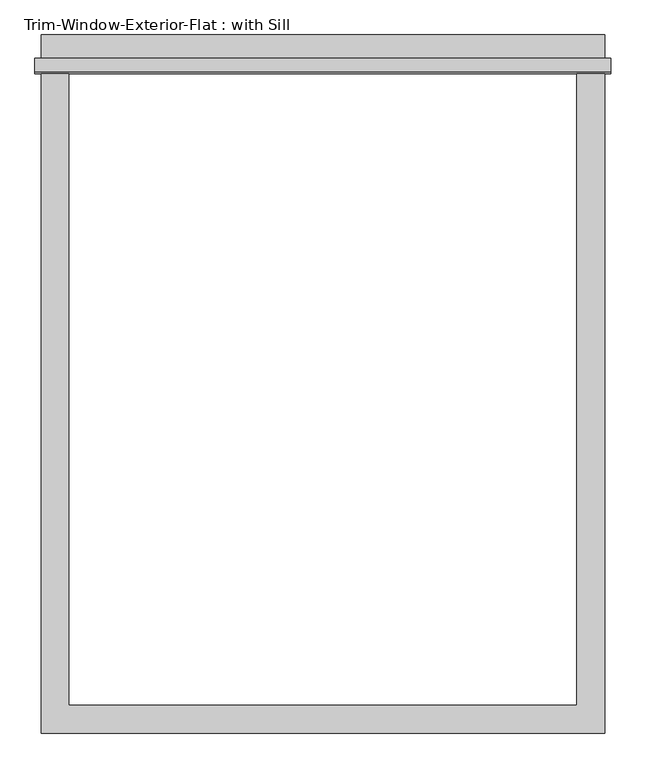
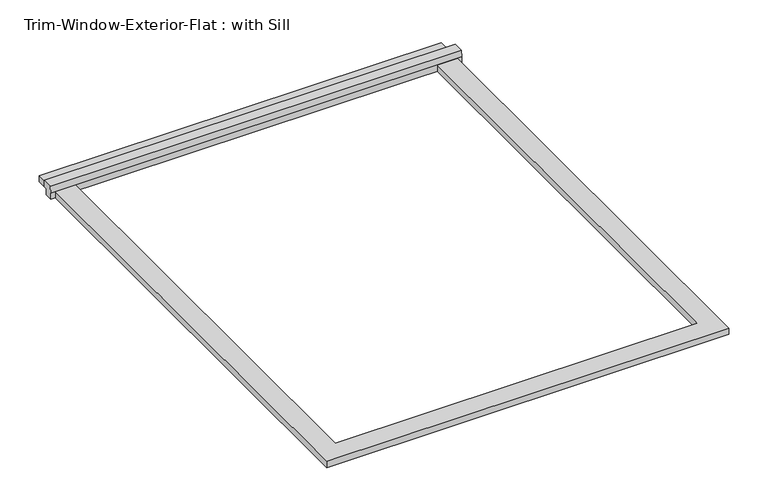
"""IFC4 building model written with IfcOpenShell, lengths in millimetres: proxy geometry, Trim-Window-Exterior-Flat : with Sill."""

import ifcopenshell
import ifcopenshell.guid

model = None  # the IFC model being written
_history = None  # IfcOwnerHistory: only IFC2X3 demands one
_inside = {}  # id of a spatial element -> (the spatial element, [elements in it])
_under = {}  # id of a project, library or spatial element -> (it, [spatial elements below it])
_declared = {}  # id of a project -> (the project, [libraries it declares])
_typed = {}  # id of a type object -> (the type object, [elements of that type])
_made_of = {}  # id of a material, layer set ... -> (it, [elements and type objects made of it])


def new_model(schema):
    """Start an empty IFC model of exactly this schema.

    Asked for "IFC4X3", IfcOpenShell would pick the latest addendum, in which some entities
    have other attributes; the version numbers below select the first issue.
    IFC2X3 requires an IfcOwnerHistory on every rooted entity: one is made here for all.
    """
    global model, _history
    if schema == "IFC4X3":
        model = ifcopenshell.file(schema_version=(4, 3, 0, 0))
    else:
        model = ifcopenshell.file(schema=schema)
    _inside.clear()
    _under.clear()
    _declared.clear()
    _typed.clear()
    _made_of.clear()
    _history = None
    if model.schema == "IFC2X3":
        org = make("IfcOrganization", Name="unknown")
        user = make(
            "IfcPersonAndOrganization",
            ThePerson=make("IfcPerson", FamilyName="unknown"),
            TheOrganization=org,
        )
        app = make(
            "IfcApplication",
            ApplicationDeveloper=org,
            Version="unknown",
            ApplicationFullName="unknown",
            ApplicationIdentifier="unknown",
        )
        _history = make(
            "IfcOwnerHistory",
            OwningUser=user,
            OwningApplication=app,
            ChangeAction="ADDED",
            CreationDate=0,
        )
    return model


def make(cls, **values):
    """One entity of the class cls with the attributes given. An attribute that is None is left unset."""
    return model.create_entity(
        cls, **{name: value for name, value in values.items() if value is not None}
    )


def rooted(cls, **values):
    """An entity with a GlobalId (a new one), such as an element, a storey or a relation."""
    return make(cls, GlobalId=ifcopenshell.guid.new(), OwnerHistory=_history, **values)


def si_unit(unit_type, name, prefix=None):
    """IfcSIUnit, for example si_unit("LENGTHUNIT", "METRE", prefix="MILLI")."""
    return make("IfcSIUnit", UnitType=unit_type, Prefix=prefix, Name=name)


def assignment(units):
    """IfcUnitAssignment: the units of a project."""
    return None if units is None else make("IfcUnitAssignment", Units=units)


def point(xyz):
    """IfcCartesianPoint."""
    return None if xyz is None else make("IfcCartesianPoint", Coordinates=xyz)


def direction(xyz):
    """IfcDirection."""
    return None if xyz is None else make("IfcDirection", DirectionRatios=xyz)


def frame(location, z_axis=None, x_axis=None):
    """IfcAxis2Placement3D, a coordinate frame: its origin and axes. An axis left out is left unset."""
    return make(
        "IfcAxis2Placement3D",
        Location=point(location),
        Axis=direction(z_axis),
        RefDirection=direction(x_axis),
    )


def origin():
    """The frame at (0, 0, 0) with its axes left unset."""
    return frame((0.0, 0.0, 0.0))


def origin_with_axes():
    """The frame at (0, 0, 0) with the z axis (0, 0, 1) and the x axis (1, 0, 0) written out."""
    return frame((0.0, 0.0, 0.0), z_axis=(0.0, 0.0, 1.0), x_axis=(1.0, 0.0, 0.0))


def place(relative_to, where):
    """IfcLocalPlacement: puts the frame where relative to a parent placement (None: the world)."""
    return make(
        "IfcLocalPlacement", PlacementRelTo=relative_to, RelativePlacement=where
    )


def context(
    kind, dimensions, precision=None, world=None, true_north=None, identifier=None
):
    """IfcGeometricRepresentationContext, for example the 3D "Model" context."""
    return make(
        "IfcGeometricRepresentationContext",
        ContextIdentifier=identifier,
        ContextType=kind,
        CoordinateSpaceDimension=dimensions,
        Precision=precision,
        WorldCoordinateSystem=world,
        TrueNorth=true_north,
    )


def project(units=None, contexts=None):
    """IfcProject with its units and contexts."""
    return rooted(
        "IfcProject",
        Name="project",
        RepresentationContexts=contexts,
        UnitsInContext=assignment(units),
    )


def spatial(cls, under=None, at=None, **own):
    """A site, building, storey or space (cls), placed at a placement, below another one or the project."""
    s = rooted(cls, ObjectPlacement=at, **own)
    if under is not None:
        _under.setdefault(under.id(), (under, []))[1].append(s)
    return s


def polyline(points):
    """IfcPolyline through the points."""
    return make("IfcPolyline", Points=[point(p) for p in points])


def outline(outer, holes=None, kind="AREA"):
    """IfcArbitraryClosedProfileDef: a profile drawn as a closed curve; with holes, ...WithVoids."""
    if holes is None:
        return make("IfcArbitraryClosedProfileDef", ProfileType=kind, OuterCurve=outer)
    return make(
        "IfcArbitraryProfileDefWithVoids",
        ProfileType=kind,
        OuterCurve=outer,
        InnerCurves=holes,
    )


def extrude(swept, where, along, depth):
    """IfcExtrudedAreaSolid: the profile swept, set in the frame where, extruded along a direction by depth."""
    return make(
        "IfcExtrudedAreaSolid",
        SweptArea=swept,
        Position=where,
        ExtrudedDirection=direction(along),
        Depth=depth,
    )


def shape(context_of_items, identifier, shape_type, items):
    """IfcShapeRepresentation: the items that make up one representation, for example the "Body"."""
    return make(
        "IfcShapeRepresentation",
        ContextOfItems=context_of_items,
        RepresentationIdentifier=identifier,
        RepresentationType=shape_type,
        Items=items,
    )


def source(mapping_origin, context_of_items, identifier, shape_type, items):
    """IfcRepresentationMap: a shape defined once, which mapped items show again and again."""
    return make(
        "IfcRepresentationMap",
        MappingOrigin=mapping_origin,
        MappedRepresentation=shape(context_of_items, identifier, shape_type, items),
    )


def transform(
    local_origin,
    x_axis=None,
    y_axis=None,
    z_axis=None,
    scale=None,
    scale2=None,
    scale3=None,
    uniform=True,
):
    """IfcCartesianTransformationOperator3D, or its non-uniform kind. x_axis, y_axis, z_axis: its Axis1, 2, 3."""
    if uniform:
        return make(
            "IfcCartesianTransformationOperator3D",
            Axis1=direction(x_axis),
            Axis2=direction(y_axis),
            LocalOrigin=point(local_origin),
            Scale=scale,
            Axis3=direction(z_axis),
        )
    return make(
        "IfcCartesianTransformationOperator3DnonUniform",
        Axis1=direction(x_axis),
        Axis2=direction(y_axis),
        LocalOrigin=point(local_origin),
        Scale=scale,
        Axis3=direction(z_axis),
        Scale2=scale2,
        Scale3=scale3,
    )


def mapped(mapping_source, mapping_target):
    """IfcMappedItem: shows the shape of a source again, moved by a transform."""
    return make(
        "IfcMappedItem", MappingSource=mapping_source, MappingTarget=mapping_target
    )


def made_of(thing, what):
    """Note that an element or type object is made of a material, layer set ...; save() writes the relation."""
    if what is not None:
        _made_of.setdefault(what.id(), (what, []))[1].append(thing)
    return thing


def element(
    cls,
    number,
    at=None,
    inside=None,
    cuts=None,
    type_object=None,
    material=None,
    context=None,
    identifier="Body",
    shape_type=None,
    held_by="IfcProductDefinitionShape",
    body=None,
    shapes=None,
    **own,
):
    """One element of the class cls, such as IfcWall. Its Tag is "e" and its number.

    at: its placement. inside: the storey or other place that contains it. cuts: it is an
    opening in that element (IfcRelVoidsElement). A single representation is given by context,
    identifier, shape_type and body (its items); several are given by shapes. held_by: the class
    of the entity that holds the representations. save() writes the other relations.
    """
    e = rooted(cls, Tag="e%d" % number, ObjectPlacement=at, **own)
    if body is not None:
        shapes = [shape(context, identifier, shape_type, body)]
    if shapes is not None:
        e.Representation = make(held_by, Representations=shapes)
    if inside is not None:
        _inside.setdefault(inside.id(), (inside, []))[1].append(e)
    if cuts is not None:
        rooted(
            "IfcRelVoidsElement", RelatingBuildingElement=cuts, RelatedOpeningElement=e
        )
    if type_object is not None:
        _typed.setdefault(type_object.id(), (type_object, []))[1].append(e)
    return made_of(e, material)


def aggregate(whole, parts):
    """IfcRelAggregates: a whole, such as a stair, and the parts it consists of."""
    return rooted("IfcRelAggregates", RelatingObject=whole, RelatedObjects=parts)


def save(model, path):
    """Write the relations noted so far, then the file.

    IfcRelAggregates (storeys below a building ...), IfcRelContainedInSpatialStructure (elements
    in a storey), IfcRelDefinesByType, IfcRelAssociatesMaterial and IfcRelDeclares: one each for
    every whole, place, type object, material and project.
    """
    for whole, parts in _under.values():
        aggregate(whole, parts)
    for where, things in _inside.values():
        rooted(
            "IfcRelContainedInSpatialStructure",
            RelatedElements=things,
            RelatingStructure=where,
        )
    for kind, things in _typed.values():
        rooted("IfcRelDefinesByType", RelatedObjects=things, RelatingType=kind)
    for what, things in _made_of.values():
        rooted("IfcRelAssociatesMaterial", RelatedObjects=things, RelatingMaterial=what)
    for by, libraries in _declared.values():
        rooted("IfcRelDeclares", RelatingContext=by, RelatedDefinitions=libraries)
    model.write(path)


def trim_window_exterior_flat_with_sill_7ce58be9(model_context):
    return source(origin(), model_context, "Body", "SweptSolid", [
        extrude(outline(polyline([(577.85, 1317.5823709), (-577.85, 1317.5823709), (-577.85, 1374.7323709), (577.85, 1374.7323709), (577.85, 1317.5823709)])), origin_with_axes(), (0.0, 0.0, 1.0), 19.05),
        extrude(outline(polyline([(1327.15, 38.1), (1327.15, 19.05), (1317.5823709, 19.05), (1317.5823709, 0.0), (1295.4, 0.0), (1295.4, 19.05), (1297.8580645, 38.1), (1327.15, 38.1)])), frame((-590.55, 0.0, 0.0), z_axis=(1.0, 0.0, 0.0), x_axis=(0.0, 1.0, 0.0)), (0.0, 0.0, 1.0), 1181.1),
        extrude(outline(polyline([(-577.85, -57.15), (-577.85, 1295.4), (-520.7, 1295.4), (-520.7, 0.0), (520.7, 0.0), (520.7, 1295.4), (577.85, 1295.4), (577.85, -57.15), (-577.85, -57.15)])), origin_with_axes(), (0.0, 0.0, 1.0), 19.05),
    ])


if __name__ == "__main__":
    model = new_model("IFC4")
    model_context = context("Model", 3, world=origin())
    ifc_project = project(units=[si_unit("LENGTHUNIT", "METRE", prefix="MILLI")], contexts=[model_context])
    site = spatial("IfcSite", under=ifc_project)
    building = spatial("IfcBuilding", under=site)
    placement = place(None, origin())
    trim_window_exterior_flat_with_sill_shape = trim_window_exterior_flat_with_sill_7ce58be9(model_context)
    element("IfcBuildingElementProxy", 1, Name="Trim-Window-Exterior-Flat : with Sill", ObjectType="Trim-Window-Exterior-Flat : with Sill", at=placement, inside=building, context=model_context, shape_type="MappedRepresentation", body=[
        mapped(trim_window_exterior_flat_with_sill_shape, transform((0.0, 0.0, 0.0), x_axis=(1.0, 0.0, 0.0), y_axis=(0.0, 1.0, 0.0), z_axis=(0.0, 0.0, 1.0))),
    ])
    save(model, "model.ifc")

# Revit data of these elements
# Type "Trim-Window-Exterior-Flat : with Sill"
#   Trim Width = 0' - 2 1/4"
#   Trim Thickness_Picture Frame = 0' - 1 1/4"
#   Trim Thickness_with Sill = 0' - 0 3/4"
#   Sill Thickness = 0' - 1 1/4"
#   Opening Width [instance default] = 2' - 0"
#   Opening Height [instance default] = 3' - 0"
#   Default Elevation = 4' - 0"
#   Sill = yes
#   Picture Frame = no
#   Trim Material [instance default] = none
# Element 1 (IfcBuildingElementProxy, "Trim-Window-Exterior-Flat : with Sill")
#   Opening Width = 3' - 5"
#   Opening Height = 4' - 3"
#   Trim Material = Clad - White
#   Materials on its faces: "Clad - White"
# Materials
#   "Clad - White": class "Wood", colour RGB 242 242 238, transparency 0, Cost = 0
